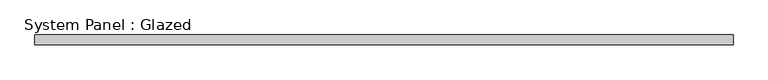
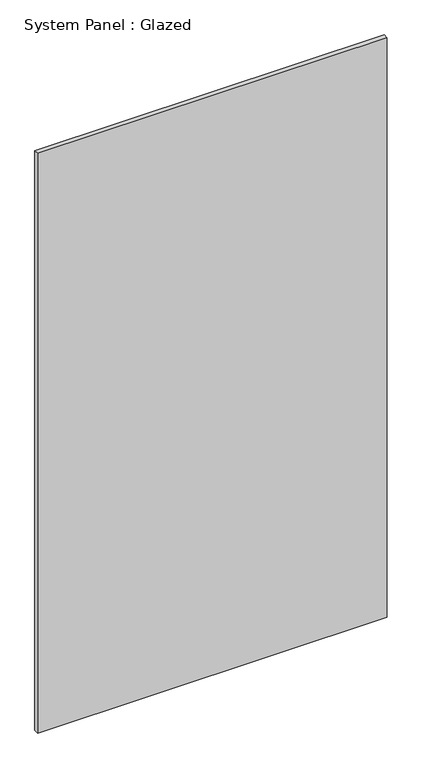
"""IFC4 building model written with IfcOpenShell, lengths in millimetres: plate geometry, System Panel : Glazed."""

from ifc_helpers import new_model, si_unit, origin, origin_with_axes, place, context, project, spatial, polyline, outline, extrude, source, transform, mapped, element, save


def system_panel_glazed_d1c08d78(model_context):
    return source(origin(), model_context, "Body", "SweptSolid", [
        extrude(outline(polyline([(904.5833334, 24.5), (-904.5833334, 24.5), (-904.5833334, 49.5), (904.5833334, 49.5), (904.5833334, 24.5)])), origin_with_axes(), (0.0, 0.0, 1.0), 3170.0),
    ])


if __name__ == "__main__":
    model = new_model("IFC4")
    model_context = context("Model", 3, world=origin())
    ifc_project = project(units=[si_unit("LENGTHUNIT", "METRE", prefix="MILLI")], contexts=[model_context])
    site = spatial("IfcSite", under=ifc_project)
    building = spatial("IfcBuilding", under=site)
    placement = place(None, origin())
    system_panel_glazed_shape = system_panel_glazed_d1c08d78(model_context)
    element("IfcPlate", 1, ObjectType="System Panel : Glazed", at=placement, inside=building, context=model_context, shape_type="MappedRepresentation", body=[
        mapped(system_panel_glazed_shape, transform((0.0, 0.0, 0.0), x_axis=(1.0, 0.0, 0.0), y_axis=(0.0, 1.0, 0.0), z_axis=(0.0, 0.0, 1.0))),
    ])
    save(model, "model.ifc")

# Revit data of these elements
# Type "System Panel : Glazed"
#   Construction Type Id = "GSP4R"
#   Analytic Construction = "1/8 in Pilkington single glazing"
#   Visual Light Transmittance = 0.9
#   Solar Heat Gain Coefficient = 0.86
#   Heat Transfer Coefficient (U) = 6.7069 W/(m²·K)
#   Define Thermal Properties by = 1
# Element 1 (IfcPlate, "System Panel : Glazed")
#   Materials on its faces: "Glass"
# Materials
#   "Glass": class "Glass", colour RGB 245 245 243, transparency 1, Description = "Soda Lime Glass", Cost = 0
